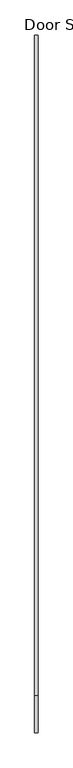
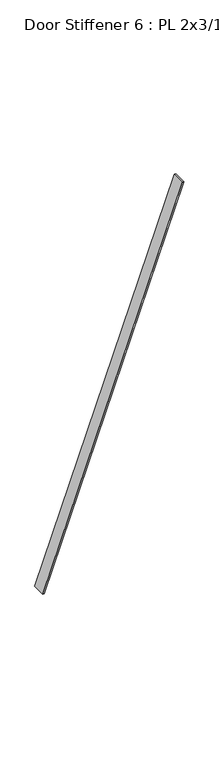
"""IFC4 building model written with IfcOpenShell, lengths in millimetres: proxy geometry, Door Stiffener 6 : PL 2x3/16."""

import ifcopenshell
import ifcopenshell.guid

model = None  # the IFC model being written
_history = None  # IfcOwnerHistory: only IFC2X3 demands one
_inside = {}  # id of a spatial element -> (the spatial element, [elements in it])
_under = {}  # id of a project, library or spatial element -> (it, [spatial elements below it])
_declared = {}  # id of a project -> (the project, [libraries it declares])
_typed = {}  # id of a type object -> (the type object, [elements of that type])
_made_of = {}  # id of a material, layer set ... -> (it, [elements and type objects made of it])


def new_model(schema):
    """Start an empty IFC model of exactly this schema.

    Asked for "IFC4X3", IfcOpenShell would pick the latest addendum, in which some entities
    have other attributes; the version numbers below select the first issue.
    IFC2X3 requires an IfcOwnerHistory on every rooted entity: one is made here for all.
    """
    global model, _history
    if schema == "IFC4X3":
        model = ifcopenshell.file(schema_version=(4, 3, 0, 0))
    else:
        model = ifcopenshell.file(schema=schema)
    _inside.clear()
    _under.clear()
    _declared.clear()
    _typed.clear()
    _made_of.clear()
    _history = None
    if model.schema == "IFC2X3":
        org = make("IfcOrganization", Name="unknown")
        user = make(
            "IfcPersonAndOrganization",
            ThePerson=make("IfcPerson", FamilyName="unknown"),
            TheOrganization=org,
        )
        app = make(
            "IfcApplication",
            ApplicationDeveloper=org,
            Version="unknown",
            ApplicationFullName="unknown",
            ApplicationIdentifier="unknown",
        )
        _history = make(
            "IfcOwnerHistory",
            OwningUser=user,
            OwningApplication=app,
            ChangeAction="ADDED",
            CreationDate=0,
        )
    return model


def make(cls, **values):
    """One entity of the class cls with the attributes given. An attribute that is None is left unset."""
    return model.create_entity(
        cls, **{name: value for name, value in values.items() if value is not None}
    )


def rooted(cls, **values):
    """An entity with a GlobalId (a new one), such as an element, a storey or a relation."""
    return make(cls, GlobalId=ifcopenshell.guid.new(), OwnerHistory=_history, **values)


def si_unit(unit_type, name, prefix=None):
    """IfcSIUnit, for example si_unit("LENGTHUNIT", "METRE", prefix="MILLI")."""
    return make("IfcSIUnit", UnitType=unit_type, Prefix=prefix, Name=name)


def assignment(units):
    """IfcUnitAssignment: the units of a project."""
    return None if units is None else make("IfcUnitAssignment", Units=units)


def point(xyz):
    """IfcCartesianPoint."""
    return None if xyz is None else make("IfcCartesianPoint", Coordinates=xyz)


def direction(xyz):
    """IfcDirection."""
    return None if xyz is None else make("IfcDirection", DirectionRatios=xyz)


def frame(location, z_axis=None, x_axis=None):
    """IfcAxis2Placement3D, a coordinate frame: its origin and axes. An axis left out is left unset."""
    return make(
        "IfcAxis2Placement3D",
        Location=point(location),
        Axis=direction(z_axis),
        RefDirection=direction(x_axis),
    )


def origin():
    """The frame at (0, 0, 0) with its axes left unset."""
    return frame((0.0, 0.0, 0.0))


def place(relative_to, where):
    """IfcLocalPlacement: puts the frame where relative to a parent placement (None: the world)."""
    return make(
        "IfcLocalPlacement", PlacementRelTo=relative_to, RelativePlacement=where
    )


def context(
    kind, dimensions, precision=None, world=None, true_north=None, identifier=None
):
    """IfcGeometricRepresentationContext, for example the 3D "Model" context."""
    return make(
        "IfcGeometricRepresentationContext",
        ContextIdentifier=identifier,
        ContextType=kind,
        CoordinateSpaceDimension=dimensions,
        Precision=precision,
        WorldCoordinateSystem=world,
        TrueNorth=true_north,
    )


def project(units=None, contexts=None):
    """IfcProject with its units and contexts."""
    return rooted(
        "IfcProject",
        Name="project",
        RepresentationContexts=contexts,
        UnitsInContext=assignment(units),
    )


def spatial(cls, under=None, at=None, **own):
    """A site, building, storey or space (cls), placed at a placement, below another one or the project."""
    s = rooted(cls, ObjectPlacement=at, **own)
    if under is not None:
        _under.setdefault(under.id(), (under, []))[1].append(s)
    return s


def polyline(points):
    """IfcPolyline through the points."""
    return make("IfcPolyline", Points=[point(p) for p in points])


def outline(outer, holes=None, kind="AREA"):
    """IfcArbitraryClosedProfileDef: a profile drawn as a closed curve; with holes, ...WithVoids."""
    if holes is None:
        return make("IfcArbitraryClosedProfileDef", ProfileType=kind, OuterCurve=outer)
    return make(
        "IfcArbitraryProfileDefWithVoids",
        ProfileType=kind,
        OuterCurve=outer,
        InnerCurves=holes,
    )


def extrude(swept, where, along, depth):
    """IfcExtrudedAreaSolid: the profile swept, set in the frame where, extruded along a direction by depth."""
    return make(
        "IfcExtrudedAreaSolid",
        SweptArea=swept,
        Position=where,
        ExtrudedDirection=direction(along),
        Depth=depth,
    )


def shape(context_of_items, identifier, shape_type, items):
    """IfcShapeRepresentation: the items that make up one representation, for example the "Body"."""
    return make(
        "IfcShapeRepresentation",
        ContextOfItems=context_of_items,
        RepresentationIdentifier=identifier,
        RepresentationType=shape_type,
        Items=items,
    )


def source(mapping_origin, context_of_items, identifier, shape_type, items):
    """IfcRepresentationMap: a shape defined once, which mapped items show again and again."""
    return make(
        "IfcRepresentationMap",
        MappingOrigin=mapping_origin,
        MappedRepresentation=shape(context_of_items, identifier, shape_type, items),
    )


def transform(
    local_origin,
    x_axis=None,
    y_axis=None,
    z_axis=None,
    scale=None,
    scale2=None,
    scale3=None,
    uniform=True,
):
    """IfcCartesianTransformationOperator3D, or its non-uniform kind. x_axis, y_axis, z_axis: its Axis1, 2, 3."""
    if uniform:
        return make(
            "IfcCartesianTransformationOperator3D",
            Axis1=direction(x_axis),
            Axis2=direction(y_axis),
            LocalOrigin=point(local_origin),
            Scale=scale,
            Axis3=direction(z_axis),
        )
    return make(
        "IfcCartesianTransformationOperator3DnonUniform",
        Axis1=direction(x_axis),
        Axis2=direction(y_axis),
        LocalOrigin=point(local_origin),
        Scale=scale,
        Axis3=direction(z_axis),
        Scale2=scale2,
        Scale3=scale3,
    )


def mapped(mapping_source, mapping_target):
    """IfcMappedItem: shows the shape of a source again, moved by a transform."""
    return make(
        "IfcMappedItem", MappingSource=mapping_source, MappingTarget=mapping_target
    )


def made_of(thing, what):
    """Note that an element or type object is made of a material, layer set ...; save() writes the relation."""
    if what is not None:
        _made_of.setdefault(what.id(), (what, []))[1].append(thing)
    return thing


def element(
    cls,
    number,
    at=None,
    inside=None,
    cuts=None,
    type_object=None,
    material=None,
    context=None,
    identifier="Body",
    shape_type=None,
    held_by="IfcProductDefinitionShape",
    body=None,
    shapes=None,
    **own,
):
    """One element of the class cls, such as IfcWall. Its Tag is "e" and its number.

    at: its placement. inside: the storey or other place that contains it. cuts: it is an
    opening in that element (IfcRelVoidsElement). A single representation is given by context,
    identifier, shape_type and body (its items); several are given by shapes. held_by: the class
    of the entity that holds the representations. save() writes the other relations.
    """
    e = rooted(cls, Tag="e%d" % number, ObjectPlacement=at, **own)
    if body is not None:
        shapes = [shape(context, identifier, shape_type, body)]
    if shapes is not None:
        e.Representation = make(held_by, Representations=shapes)
    if inside is not None:
        _inside.setdefault(inside.id(), (inside, []))[1].append(e)
    if cuts is not None:
        rooted(
            "IfcRelVoidsElement", RelatingBuildingElement=cuts, RelatedOpeningElement=e
        )
    if type_object is not None:
        _typed.setdefault(type_object.id(), (type_object, []))[1].append(e)
    return made_of(e, material)


def aggregate(whole, parts):
    """IfcRelAggregates: a whole, such as a stair, and the parts it consists of."""
    return rooted("IfcRelAggregates", RelatingObject=whole, RelatedObjects=parts)


def save(model, path):
    """Write the relations noted so far, then the file.

    IfcRelAggregates (storeys below a building ...), IfcRelContainedInSpatialStructure (elements
    in a storey), IfcRelDefinesByType, IfcRelAssociatesMaterial and IfcRelDeclares: one each for
    every whole, place, type object, material and project.
    """
    for whole, parts in _under.values():
        aggregate(whole, parts)
    for where, things in _inside.values():
        rooted(
            "IfcRelContainedInSpatialStructure",
            RelatedElements=things,
            RelatingStructure=where,
        )
    for kind, things in _typed.values():
        rooted("IfcRelDefinesByType", RelatedObjects=things, RelatingType=kind)
    for what, things in _made_of.values():
        rooted("IfcRelAssociatesMaterial", RelatedObjects=things, RelatingMaterial=what)
    for by, libraries in _declared.values():
        rooted("IfcRelDeclares", RelatingContext=by, RelatedDefinitions=libraries)
    model.write(path)


def door_stiffener_6_pl_2x3_16_59935e34(model_context):
    return source(origin(), model_context, "Body", "SweptSolid", [
        extrude(outline(polyline([(-536208.5749853, 2400.3), (-535246.0163841, 88.9), (-535301.0452829, 88.9), (-536263.6038841, 2400.3), (-536208.5749853, 2400.3)])), frame((587403.9934739, 0.0, 0.0), z_axis=(1.0, 0.0, 0.0), x_axis=(0.0, 1.0, 0.0)), (0.0, 0.0, 1.0), 4.7625),
    ])


if __name__ == "__main__":
    model = new_model("IFC4")
    model_context = context("Model", 3, world=origin())
    ifc_project = project(units=[si_unit("LENGTHUNIT", "METRE", prefix="MILLI")], contexts=[model_context])
    site = spatial("IfcSite", under=ifc_project)
    building = spatial("IfcBuilding", under=site)
    placement = place(None, origin())
    door_stiffener_6_pl_2x3_16_shape = door_stiffener_6_pl_2x3_16_59935e34(model_context)
    element("IfcBuildingElementProxy", 1, Name="Door Stiffener 6 : PL 2x3/16", ObjectType="Door Stiffener 6 : PL 2x3/16", at=placement, inside=building, context=model_context, shape_type="MappedRepresentation", body=[
        mapped(door_stiffener_6_pl_2x3_16_shape, transform((0.0, 0.0, 0.0), x_axis=(1.0, 0.0, 0.0), y_axis=(0.0, 1.0, 0.0), z_axis=(0.0, 0.0, 1.0))),
    ])
    save(model, "model.ifc")

# Revit data of these elements
# Element 1 (IfcBuildingElementProxy, "Door Stiffener 6 : PL 2x3/16")
#   Materials on its faces: "2\"X3/16\" GALV. STL BAR STOCK"
# Materials
#   "2\"X3/16\" GALV. STL BAR STOCK": class "Generic", colour RGB 211 211 207, transparency 0, Cost = 0
